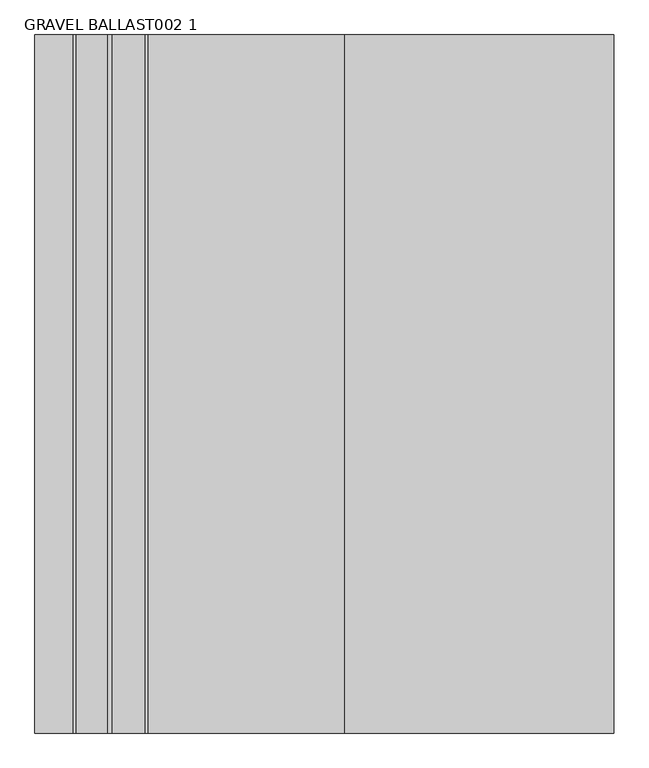
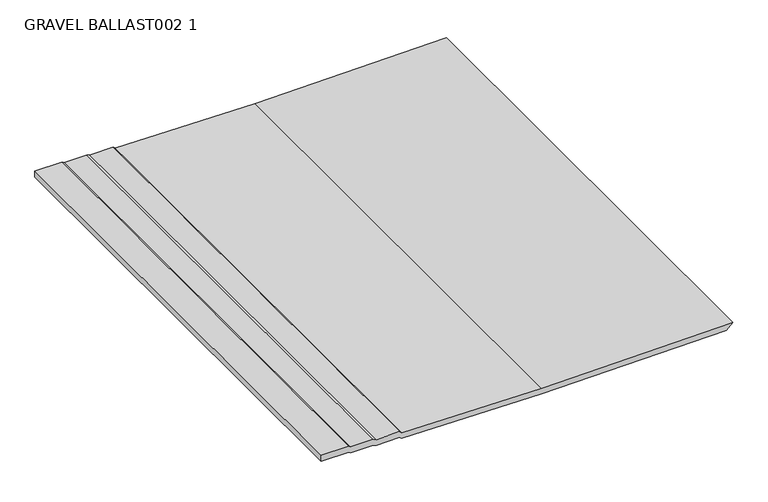
"""IFC4 building model written with IfcOpenShell, lengths in millimetres: proxy geometry, GRAVEL BALLAST002 1 : GRAVEL BALLAST002 15468."""

from ifc_helpers import new_model, si_unit, frame, origin, place, context, project, spatial, polyline, outline, extrude, source, transform, mapped, element, save


def gravel_ballast002_1_deb63274(model_context):
    return source(origin(), model_context, "Body", "SweptSolid", [
        extrude(outline(polyline([(40274.2359465, -2672.3662777), (40269.9546965, -2663.6558285), (40269.9546965, -2573.0689144), (40264.2272345, -2560.2242751), (40265.8726652, -2466.2725277), (40258.462509, -2457.9990902), (40250.243759, -1894.9286556), (40261.546875, -1149.4367676), (40286.2851563, -1123.4630127), (40274.9820403, -1894.9286556), (40283.2007903, -2457.9990902), (40290.6109465, -2466.2725277), (40288.9655158, -2560.2242751), (40294.6929778, -2573.0689144), (40294.6929778, -2663.6558285), (40298.9742278, -2672.3662777), (40298.9742278, -2781.8657894), (40274.2359465, -2781.8657894), (40274.2359465, -2672.3662777)])), frame((0.0, -1052.6406573, 0.0), z_axis=(0.0, 1.0, 0.0), x_axis=(0.0, 0.0, 1.0)), (0.0, 0.0, 1.0), 2000.0),
    ])


if __name__ == "__main__":
    model = new_model("IFC4")
    model_context = context("Model", 3, world=origin())
    ifc_project = project(units=[si_unit("LENGTHUNIT", "METRE", prefix="MILLI")], contexts=[model_context])
    site = spatial("IfcSite", under=ifc_project)
    building = spatial("IfcBuilding", under=site)
    placement = place(None, origin())
    gravel_ballast002_1_shape = gravel_ballast002_1_deb63274(model_context)
    element("IfcBuildingElementProxy", 1, Name="GRAVEL BALLAST002 1 : GRAVEL BALLAST002 15468", ObjectType="GRAVEL BALLAST002 1 : GRAVEL BALLAST002 15468", at=placement, inside=building, context=model_context, shape_type="MappedRepresentation", body=[
        mapped(gravel_ballast002_1_shape, transform((0.0, 0.0, 0.0), x_axis=(1.0, 0.0, 0.0), y_axis=(0.0, 1.0, 0.0), z_axis=(0.0, 0.0, 1.0))),
    ])
    save(model, "model.ifc")

# Revit data of these elements
# Type "GRAVEL BALLAST002 1 : GRAVEL BALLAST002 15468"
#   NameOverride = "GRAVEL BALLAST002"
# Element 1 (IfcBuildingElementProxy, "GRAVEL BALLAST002 1 : GRAVEL BALLAST002 15468")
#   Materials on its faces: "GRAVEL BALLAST"
# Materials
#   "GRAVEL BALLAST": class "Unassigned", colour RGB 128 128 128, transparency 0, Cost = 0
